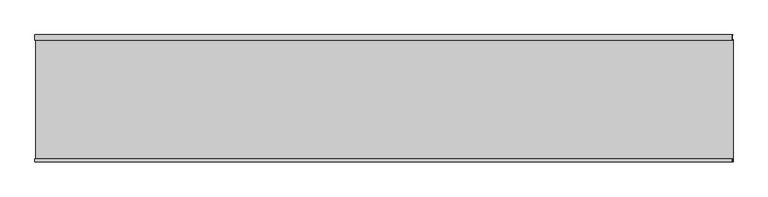
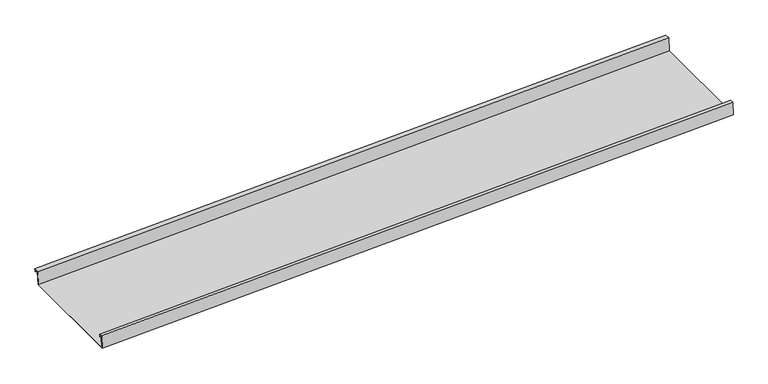
"""IFC4 building model written with IfcOpenShell, lengths in millimetres: proxy geometry, Generic Models 2:Generic Models 2:310765:Generic Models 2:310765 : Generic Models 2:Generic Models 2:310765:21 : Generic Models 2:Generic Models 2:310765:Generic Models 2:310765 : Generic Models 2:Generic Models 2:310765:300385."""

from ifc_helpers import new_model, si_unit, frame, origin, place, context, project, spatial, polyline, outline, extrude, source, transform, mapped, element, save


def generic_models_4fe5e831(model_context):
    return source(origin(), model_context, "Body", "SweptSolid", [
        extrude(outline(polyline([(1.5875, 0.0), (1.5875, 50.8), (407.9875, 50.8), (407.9875, 1.5875), (396.875, 1.5875), (396.875, 11.1125), (398.4625, 11.1125), (398.4625, 3.175), (406.4, 3.175), (406.4, 49.2125), (3.175, 49.2125), (3.175, -1.5874999), (-14.2875, -1.5874999), (-14.2875, 9.525), (-12.7, 9.525), (-12.7, 0.0), (1.5875, 0.0)])), frame((558011.7406069, -578931.1059673, 3902.662383), z_axis=(0.9991330730923568, 0.0, 0.041630544712067834), x_axis=(0.0, -1.0, 0.0)), (0.0, 0.0, 1.0), 2310.9023377),
    ])


if __name__ == "__main__":
    model = new_model("IFC4")
    model_context = context("Model", 3, world=origin())
    ifc_project = project(units=[si_unit("LENGTHUNIT", "METRE", prefix="MILLI")], contexts=[model_context])
    site = spatial("IfcSite", under=ifc_project)
    building = spatial("IfcBuilding", under=site)
    placement = place(None, origin())
    generic_models_shape = generic_models_4fe5e831(model_context)
    element("IfcBuildingElementProxy", 1, Name="Generic Models 2:Generic Models 2:310765:Generic Models 2:310765 : Generic Models 2:Generic Models 2:310765:21 : Generic Models 2:Generic Models 2:310765:Generic Models 2:310765 : Generic Models 2:Generic Models 2:310765:300385", ObjectType="Generic Models 2:Generic Models 2:310765:Generic Models 2:310765 : Generic Models 2:Generic Models 2:310765:21 : Generic Models 2:Generic Models 2:310765:Generic Models 2:310765 : Generic Models 2:Generic Models 2:310765:300385", at=placement, inside=building, context=model_context, shape_type="MappedRepresentation", body=[
        mapped(generic_models_shape, transform((0.0, 0.0, 0.0), x_axis=(1.0, 0.0, 0.0), y_axis=(0.0, 1.0, 0.0), z_axis=(0.0, 0.0, 1.0))),
    ])
    save(model, "model.ifc")

# Revit data of these elements
# Type "Generic Models 2:Generic Models 2:310765:Generic Models 2:310765 : Generic Models 2:Generic Models 2:310765:21 : Generic Models 2:Generic Models 2:310765:Generic Models 2:310765 : Generic Models 2:Generic Models 2:310765:300385"
#   NameOverride = "Generic Models 2:Generic Models 2:310765:Generic Models 2:310765 : Generic Models 2:Generic Models 2:310765:300385"
#   ObjectTypeOverride = "Generic Models 2:310765 : Generic Models 2:Generic Models 2:310765"
#   Reference = "Generic Models 2"
#   Tag = "300385"
# Element 1 (IfcBuildingElementProxy, "Generic Models 2:Generic Models 2:310765:Generic Models 2:310765 : Generic Models 2:Generic Models 2:310765:21 : Generic Models 2:Generic Models 2:310765:Generic Models 2:310765 : Generic Models 2:Generic Models 2:310765:300385")
#   Materials on its faces: "THERMAL BROKEN ALUMINUM STOREFRONT FOR POLYCARBONATE"
# Materials
#   "THERMAL BROKEN ALUMINUM STOREFRONT FOR POLYCARBONATE": class "Unassigned", colour RGB 244 244 244, transparency 0, Keynote = "M07611300.01", Cost = 0
